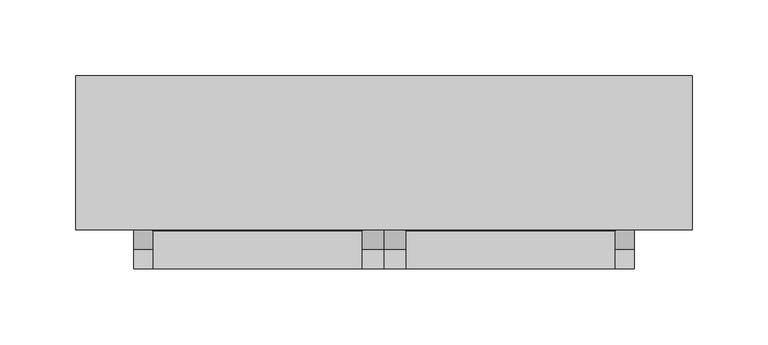
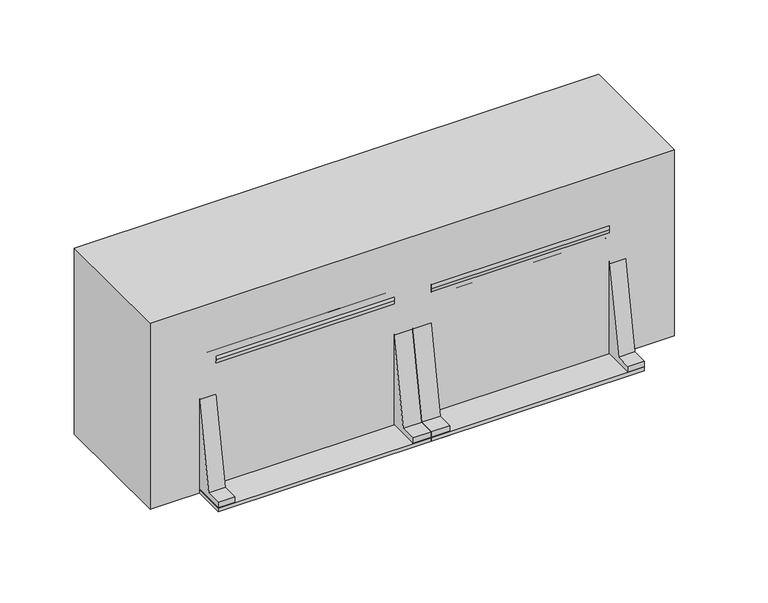
"""IFC4 building model written with IfcOpenShell, lengths in millimetres: proxy geometry, A5202 - Dispenser,Toilet Paper W Utility Shelf, SS, 2-Roll : A5202 - Dispenser,Toilet Paper W Utility Shelf, SS, 2-Roll."""

import ifcopenshell
import ifcopenshell.guid

model = None  # the IFC model being written
_history = None  # IfcOwnerHistory: only IFC2X3 demands one
_inside = {}  # id of a spatial element -> (the spatial element, [elements in it])
_under = {}  # id of a project, library or spatial element -> (it, [spatial elements below it])
_declared = {}  # id of a project -> (the project, [libraries it declares])
_typed = {}  # id of a type object -> (the type object, [elements of that type])
_made_of = {}  # id of a material, layer set ... -> (it, [elements and type objects made of it])


def new_model(schema):
    """Start an empty IFC model of exactly this schema.

    Asked for "IFC4X3", IfcOpenShell would pick the latest addendum, in which some entities
    have other attributes; the version numbers below select the first issue.
    IFC2X3 requires an IfcOwnerHistory on every rooted entity: one is made here for all.
    """
    global model, _history
    if schema == "IFC4X3":
        model = ifcopenshell.file(schema_version=(4, 3, 0, 0))
    else:
        model = ifcopenshell.file(schema=schema)
    _inside.clear()
    _under.clear()
    _declared.clear()
    _typed.clear()
    _made_of.clear()
    _history = None
    if model.schema == "IFC2X3":
        org = make("IfcOrganization", Name="unknown")
        user = make(
            "IfcPersonAndOrganization",
            ThePerson=make("IfcPerson", FamilyName="unknown"),
            TheOrganization=org,
        )
        app = make(
            "IfcApplication",
            ApplicationDeveloper=org,
            Version="unknown",
            ApplicationFullName="unknown",
            ApplicationIdentifier="unknown",
        )
        _history = make(
            "IfcOwnerHistory",
            OwningUser=user,
            OwningApplication=app,
            ChangeAction="ADDED",
            CreationDate=0,
        )
    return model


def make(cls, **values):
    """One entity of the class cls with the attributes given. An attribute that is None is left unset."""
    return model.create_entity(
        cls, **{name: value for name, value in values.items() if value is not None}
    )


def rooted(cls, **values):
    """An entity with a GlobalId (a new one), such as an element, a storey or a relation."""
    return make(cls, GlobalId=ifcopenshell.guid.new(), OwnerHistory=_history, **values)


def si_unit(unit_type, name, prefix=None):
    """IfcSIUnit, for example si_unit("LENGTHUNIT", "METRE", prefix="MILLI")."""
    return make("IfcSIUnit", UnitType=unit_type, Prefix=prefix, Name=name)


def assignment(units):
    """IfcUnitAssignment: the units of a project."""
    return None if units is None else make("IfcUnitAssignment", Units=units)


def point(xyz):
    """IfcCartesianPoint."""
    return None if xyz is None else make("IfcCartesianPoint", Coordinates=xyz)


def direction(xyz):
    """IfcDirection."""
    return None if xyz is None else make("IfcDirection", DirectionRatios=xyz)


def frame(location, z_axis=None, x_axis=None):
    """IfcAxis2Placement3D, a coordinate frame: its origin and axes. An axis left out is left unset."""
    return make(
        "IfcAxis2Placement3D",
        Location=point(location),
        Axis=direction(z_axis),
        RefDirection=direction(x_axis),
    )


def frame_2d(location, x_axis=None):
    """IfcAxis2Placement2D, a coordinate frame in the plane: its origin and x axis."""
    return make(
        "IfcAxis2Placement2D", Location=point(location), RefDirection=direction(x_axis)
    )


def origin():
    """The frame at (0, 0, 0) with its axes left unset."""
    return frame((0.0, 0.0, 0.0))


def origin_with_axes():
    """The frame at (0, 0, 0) with the z axis (0, 0, 1) and the x axis (1, 0, 0) written out."""
    return frame((0.0, 0.0, 0.0), z_axis=(0.0, 0.0, 1.0), x_axis=(1.0, 0.0, 0.0))


def place(relative_to, where):
    """IfcLocalPlacement: puts the frame where relative to a parent placement (None: the world)."""
    return make(
        "IfcLocalPlacement", PlacementRelTo=relative_to, RelativePlacement=where
    )


def context(
    kind, dimensions, precision=None, world=None, true_north=None, identifier=None
):
    """IfcGeometricRepresentationContext, for example the 3D "Model" context."""
    return make(
        "IfcGeometricRepresentationContext",
        ContextIdentifier=identifier,
        ContextType=kind,
        CoordinateSpaceDimension=dimensions,
        Precision=precision,
        WorldCoordinateSystem=world,
        TrueNorth=true_north,
    )


def project(units=None, contexts=None):
    """IfcProject with its units and contexts."""
    return rooted(
        "IfcProject",
        Name="project",
        RepresentationContexts=contexts,
        UnitsInContext=assignment(units),
    )


def spatial(cls, under=None, at=None, **own):
    """A site, building, storey or space (cls), placed at a placement, below another one or the project."""
    s = rooted(cls, ObjectPlacement=at, **own)
    if under is not None:
        _under.setdefault(under.id(), (under, []))[1].append(s)
    return s


def polyline(points):
    """IfcPolyline through the points."""
    return make("IfcPolyline", Points=[point(p) for p in points])


def circle_curve(where, radius):
    """IfcCircle in the frame where."""
    return make("IfcCircle", Position=where, Radius=radius)


def trimmed(basis, trim1, trim2, sense, master):
    """IfcTrimmedCurve: the piece of a basis curve between two trims."""
    return make(
        "IfcTrimmedCurve",
        BasisCurve=basis,
        Trim1=trim1,
        Trim2=trim2,
        SenseAgreement=sense,
        MasterRepresentation=master,
    )


def segment(curve, same_sense, transition):
    """IfcCompositeCurveSegment."""
    return make(
        "IfcCompositeCurveSegment",
        Transition=transition,
        SameSense=same_sense,
        ParentCurve=curve,
    )


def composite_curve(segments, self_intersect=None):
    """IfcCompositeCurve: segments joined end to end."""
    return make("IfcCompositeCurve", Segments=segments, SelfIntersect=self_intersect)


def outline(outer, holes=None, kind="AREA"):
    """IfcArbitraryClosedProfileDef: a profile drawn as a closed curve; with holes, ...WithVoids."""
    if holes is None:
        return make("IfcArbitraryClosedProfileDef", ProfileType=kind, OuterCurve=outer)
    return make(
        "IfcArbitraryProfileDefWithVoids",
        ProfileType=kind,
        OuterCurve=outer,
        InnerCurves=holes,
    )


def extrude(swept, where, along, depth):
    """IfcExtrudedAreaSolid: the profile swept, set in the frame where, extruded along a direction by depth."""
    return make(
        "IfcExtrudedAreaSolid",
        SweptArea=swept,
        Position=where,
        ExtrudedDirection=direction(along),
        Depth=depth,
    )


def faces_of(points, faces, orient=None, outer=None):
    """IfcFace entities. A face is a list of loops; a loop is a list of indices into points, from 0.

    orient and outer hold one flag for each loop. By default every Orientation is true, the
    first loop of a face is its IfcFaceOuterBound and the others are IfcFaceBound.
    """
    made = []
    for i, loops in enumerate(faces):
        bounds = []
        for j, loop in enumerate(loops):
            is_outer = j == 0 if outer is None else outer[i][j]
            bounds.append(
                make(
                    "IfcFaceOuterBound" if is_outer else "IfcFaceBound",
                    Bound=make("IfcPolyLoop", Polygon=[points[k] for k in loop]),
                    Orientation=True if orient is None else orient[i][j],
                )
            )
        made.append(make("IfcFace", Bounds=bounds))
    return made


def faceted_brep(points, faces, orient=None, outer=None, voids=None):
    """IfcFacetedBrep: a solid bounded by flat faces; with voids (closed shells), ...WithVoids."""
    shared = [point(p) for p in points]
    hull = make("IfcClosedShell", CfsFaces=faces_of(shared, faces, orient, outer))
    if voids is None:
        return make("IfcFacetedBrep", Outer=hull)
    return make(
        "IfcFacetedBrepWithVoids",
        Outer=hull,
        Voids=[
            make(cls, CfsFaces=faces_of(shared, fs, o, b)) for cls, fs, o, b in voids
        ],
    )


def shape(context_of_items, identifier, shape_type, items):
    """IfcShapeRepresentation: the items that make up one representation, for example the "Body"."""
    return make(
        "IfcShapeRepresentation",
        ContextOfItems=context_of_items,
        RepresentationIdentifier=identifier,
        RepresentationType=shape_type,
        Items=items,
    )


def source(mapping_origin, context_of_items, identifier, shape_type, items):
    """IfcRepresentationMap: a shape defined once, which mapped items show again and again."""
    return make(
        "IfcRepresentationMap",
        MappingOrigin=mapping_origin,
        MappedRepresentation=shape(context_of_items, identifier, shape_type, items),
    )


def transform(
    local_origin,
    x_axis=None,
    y_axis=None,
    z_axis=None,
    scale=None,
    scale2=None,
    scale3=None,
    uniform=True,
):
    """IfcCartesianTransformationOperator3D, or its non-uniform kind. x_axis, y_axis, z_axis: its Axis1, 2, 3."""
    if uniform:
        return make(
            "IfcCartesianTransformationOperator3D",
            Axis1=direction(x_axis),
            Axis2=direction(y_axis),
            LocalOrigin=point(local_origin),
            Scale=scale,
            Axis3=direction(z_axis),
        )
    return make(
        "IfcCartesianTransformationOperator3DnonUniform",
        Axis1=direction(x_axis),
        Axis2=direction(y_axis),
        LocalOrigin=point(local_origin),
        Scale=scale,
        Axis3=direction(z_axis),
        Scale2=scale2,
        Scale3=scale3,
    )


def mapped(mapping_source, mapping_target):
    """IfcMappedItem: shows the shape of a source again, moved by a transform."""
    return make(
        "IfcMappedItem", MappingSource=mapping_source, MappingTarget=mapping_target
    )


def made_of(thing, what):
    """Note that an element or type object is made of a material, layer set ...; save() writes the relation."""
    if what is not None:
        _made_of.setdefault(what.id(), (what, []))[1].append(thing)
    return thing


def element(
    cls,
    number,
    at=None,
    inside=None,
    cuts=None,
    type_object=None,
    material=None,
    context=None,
    identifier="Body",
    shape_type=None,
    held_by="IfcProductDefinitionShape",
    body=None,
    shapes=None,
    **own,
):
    """One element of the class cls, such as IfcWall. Its Tag is "e" and its number.

    at: its placement. inside: the storey or other place that contains it. cuts: it is an
    opening in that element (IfcRelVoidsElement). A single representation is given by context,
    identifier, shape_type and body (its items); several are given by shapes. held_by: the class
    of the entity that holds the representations. save() writes the other relations.
    """
    e = rooted(cls, Tag="e%d" % number, ObjectPlacement=at, **own)
    if body is not None:
        shapes = [shape(context, identifier, shape_type, body)]
    if shapes is not None:
        e.Representation = make(held_by, Representations=shapes)
    if inside is not None:
        _inside.setdefault(inside.id(), (inside, []))[1].append(e)
    if cuts is not None:
        rooted(
            "IfcRelVoidsElement", RelatingBuildingElement=cuts, RelatedOpeningElement=e
        )
    if type_object is not None:
        _typed.setdefault(type_object.id(), (type_object, []))[1].append(e)
    return made_of(e, material)


def aggregate(whole, parts):
    """IfcRelAggregates: a whole, such as a stair, and the parts it consists of."""
    return rooted("IfcRelAggregates", RelatingObject=whole, RelatedObjects=parts)


def save(model, path):
    """Write the relations noted so far, then the file.

    IfcRelAggregates (storeys below a building ...), IfcRelContainedInSpatialStructure (elements
    in a storey), IfcRelDefinesByType, IfcRelAssociatesMaterial and IfcRelDeclares: one each for
    every whole, place, type object, material and project.
    """
    for whole, parts in _under.values():
        aggregate(whole, parts)
    for where, things in _inside.values():
        rooted(
            "IfcRelContainedInSpatialStructure",
            RelatedElements=things,
            RelatingStructure=where,
        )
    for kind, things in _typed.values():
        rooted("IfcRelDefinesByType", RelatedObjects=things, RelatingType=kind)
    for what, things in _made_of.values():
        rooted("IfcRelAssociatesMaterial", RelatedObjects=things, RelatingMaterial=what)
    for by, libraries in _declared.values():
        rooted("IfcRelDeclares", RelatingContext=by, RelatedDefinitions=libraries)
    model.write(path)


def specialty_equipment_d6a35412(model_context):
    return source(origin(), model_context, "Body", "SolidModel", [
        extrude(outline(polyline([(203.2, 0.0), (203.2, -101.6), (-203.2, -101.6), (-203.2, 0.0), (203.2, 0.0)])), origin_with_axes(), (0.0, 0.0, 1.0), 152.4),
        faceted_brep([(152.4, -3.175, 3.175), (-152.4, -3.175, 3.175), (-152.4, -12.7, 3.175), (152.4, -12.7, 3.175), (165.1, -12.7, 149.225), (165.1, 0.0, 149.225), (-165.1, 0.0, 149.225), (-165.1, -12.7, 149.225), (165.1, -12.7, 0.0), (-165.1, -12.7, 0.0), (-165.1, 0.0, 0.0), (165.1, 0.0, 0.0), (-152.4, -12.7, 145.6205323), (152.4, -12.7, 145.6205323), (152.4, -3.175, 145.6205323), (-152.4, -3.175, 145.6205323)], [[[0, 1, 2, 3]], [[4, 5, 6, 7]], [[8, 9, 10, 11]], [[5, 4, 8, 11]], [[6, 5, 11, 10]], [[7, 6, 10, 9]], [[4, 7, 9, 8], [12, 13, 3, 2]], [[14, 15, 1, 0]], [[15, 14, 13, 12]], [[1, 15, 12, 2]], [[14, 0, 3, 13]]]),
        extrude(outline(polyline([(0.0, -12.7), (165.1, -12.7), (165.1, -127.2036203), (0.0, -127.2036203), (0.0, -12.7)])), origin_with_axes(), (0.0, 0.0, 1.0), 3.175),
        extrude(outline(polyline([(-124.0286203, 0.0), (0.0, 0.0), (0.0, -7.9375), (-12.7, -7.9375), (-33.2613189, -120.65), (-114.5036203, -120.65), (-114.5036203, -3.175), (-124.0286203, -3.175), (-124.0286203, 0.0)])), frame((0.0, -127.2036203, 0.0), z_axis=(1.0, 1.020266240683039e-12, 0.0), x_axis=(1.020266240683039e-12, -1.0, 0.0)), (0.0, 0.0, 1.0), 14.2875),
        extrude(outline(polyline([(-114.5036203, 0.0), (0.0, 0.0), (0.0, -7.9375), (-12.7, -7.9375), (-33.2613189, -120.65), (-114.5036203, -120.65), (-114.5036203, 0.0)])), frame((152.4, -127.2036203, 0.0), z_axis=(1.0, 1.020266240683039e-12, 0.0), x_axis=(1.020266240683039e-12, -1.0, 0.0)), (0.0, 0.0, 1.0), 12.7),
        extrude(outline(polyline([(0.0, -12.7), (0.0, -127.2036203), (-165.1, -127.2036203), (-165.1, -12.7), (0.0, -12.7)])), origin_with_axes(), (0.0, 0.0, 1.0), 3.175),
        extrude(outline(polyline([(0.0, 0.0), (0.0, -124.0286203), (-7.9375, -124.0286203), (-7.9375, -111.3286203), (-120.65, -90.7673014), (-120.65, -9.525), (-3.175, -9.525), (-3.175, 0.0), (0.0, 0.0)])), frame((-14.2875, -3.175, 0.0), z_axis=(1.0, 1.0170616637688368e-12, 0.0), x_axis=(0.0, 0.0, -1.0)), (0.0, 0.0, 1.0), 14.2875),
        extrude(outline(polyline([(0.0, 0.0), (0.0, -114.5036203), (-7.9375, -114.5036203), (-7.9375, -101.8036203), (-120.65, -81.2423014), (-120.65, 0.0), (0.0, 0.0)])), frame((-165.1, -12.7, 0.0), z_axis=(1.0, 1.0170616637688368e-12, 0.0), x_axis=(0.0, 0.0, -1.0)), (0.0, 0.0, 1.0), 12.7),
        extrude(outline(composite_curve([segment(trimmed(circle_curve(frame_2d((0.0, -13.382926)), 13.382926), [point((0.0, -26.765852))], [point((0.0, 0.0))], False, "CARTESIAN"), True, "CONTINUOUS"), segment(trimmed(circle_curve(frame_2d((0.0, -13.382926)), 13.382926), [point((0.0, 0.0))], [point((0.0, -26.765852))], False, "CARTESIAN"), True, "CONTINUOUS")], self_intersect=False)), frame((14.2875, -75.517074, 105.1171268), z_axis=(1.0, 1.020266240683039e-12, 0.0), x_axis=(0.0, 0.0, -1.0)), (0.0, 0.0, 1.0), 138.1125),
        extrude(outline(composite_curve([segment(trimmed(circle_curve(frame_2d((0.0, -1.8851296)), 1.8851296), [point((0.0, -3.7702592))], [point((0.0, 0.0))], False, "CARTESIAN"), True, "CONTINUOUS"), segment(trimmed(circle_curve(frame_2d((0.0, -1.8851296)), 1.8851296), [point((0.0, 0.0))], [point((0.0, -3.7702592))], False, "CARTESIAN"), True, "CONTINUOUS")], self_intersect=False)), frame((14.2875, -88.9, 107.0022564), z_axis=(1.0, 1.018725182543629e-12, 0.0), x_axis=(-1.018725182543629e-12, 1.0, 0.0)), (0.0, 0.0, 1.0), 138.1125),
        extrude(outline(composite_curve([segment(trimmed(circle_curve(frame_2d((0.0, -13.382926)), 13.382926), [point((0.0, -26.765852))], [point((0.0, 0.0))], False, "CARTESIAN"), True, "CONTINUOUS"), segment(trimmed(circle_curve(frame_2d((0.0, -13.382926)), 13.382926), [point((0.0, 0.0))], [point((0.0, -26.765852))], False, "CARTESIAN"), True, "CONTINUOUS")], self_intersect=False)), frame((-152.4, -75.517074, 105.1171268), z_axis=(1.0, 1.0170616637688368e-12, 0.0), x_axis=(0.0, 0.0, -1.0)), (0.0, 0.0, 1.0), 138.1125),
        extrude(outline(composite_curve([segment(trimmed(circle_curve(frame_2d((0.0, -1.8851296)), 1.8851296), [point((0.0, -3.7702592))], [point((0.0, 0.0))], False, "CARTESIAN"), True, "CONTINUOUS"), segment(trimmed(circle_curve(frame_2d((0.0, -1.8851296)), 1.8851296), [point((0.0, 0.0))], [point((0.0, -3.7702592))], False, "CARTESIAN"), True, "CONTINUOUS")], self_intersect=False)), frame((-152.4, -88.9, 107.0022564), z_axis=(1.0, 1.0186027219082467e-12, 0.0), x_axis=(-1.0186027219082467e-12, 1.0, 0.0)), (0.0, 0.0, 1.0), 138.1125),
    ])


if __name__ == "__main__":
    model = new_model("IFC4")
    model_context = context("Model", 3, world=origin())
    ifc_project = project(units=[si_unit("LENGTHUNIT", "METRE", prefix="MILLI")], contexts=[model_context])
    site = spatial("IfcSite", under=ifc_project)
    building = spatial("IfcBuilding", under=site)
    placement = place(None, origin())
    specialty_equipment_shape = specialty_equipment_d6a35412(model_context)
    element("IfcBuildingElementProxy", 1, Name="A5202 - Dispenser,Toilet Paper W Utility Shelf, SS, 2-Roll : A5202 - Dispenser,Toilet Paper W Utility Shelf, SS, 2-Roll", ObjectType="A5202 - Dispenser,Toilet Paper W Utility Shelf, SS, 2-Roll : A5202 - Dispenser,Toilet Paper W Utility Shelf, SS, 2-Roll", at=placement, inside=building, context=model_context, shape_type="MappedRepresentation", body=[
        mapped(specialty_equipment_shape, transform((0.0, 0.0, 0.0), x_axis=(1.0, 0.0, 0.0), y_axis=(0.0, 1.0, 0.0), z_axis=(0.0, 0.0, 1.0))),
    ])
    save(model, "model.ifc")

# Revit data of these elements
# Type "A5202 - Dispenser,Toilet Paper W Utility Shelf, SS, 2-Roll : A5202 - Dispenser,Toilet Paper W Utility Shelf, SS, 2-Roll"
#   Watts2 = "0"
#   Watts1 = "0"
#   Unit_Issue = "EA"
#   UTIL_6_Misc = "-"
#   UTIL_5_NonMedGas = "-"
#   UTIL_4_MiscGas = "-"
#   UTIL_3_MedGas = "-"
#   UTIL_2_Elec = "-"
#   UTIL_1_WaterDrain = "-"
#   Nomenclature = "Dispenser,Toilet Paper w/Utility Shelf, SS, 2-Roll"
#   NSN = "4510"
#   Location [instance default] = ""
#   JSN = "A5202"
#   Fund_Source_VA = "-"
#   Fund_Source_Navy = "-"
#   Fund_Source_Army = "-"
#   Fund_Source_AF = "-"
#   ELEC_Volts2 = "0"
#   ELEC_Volts1 = "0"
#   ELEC_Phase2 = "0"
#   ELEC_Phase1 = "0"
#   ELEC_HertzSwitch = "0"
#   ELEC_HertzDependent = "0"
#   ELEC_Hertz = "0"
#   ELEC_Amps2 = "0"
#   ELEC_Amps1 = "0"
#   DetailDescription = "A concealed surface mounted, double roll, satin finish stainless steel, combination toilet tissue dispenser and utility shelf (minimum 5\" depth). Unit accommodates two standard-core toilet tissue rolls through 6\" in diameter. Spindles are chrome plated plastic with a heavyduty internal spring and turn freely for non-controlled delivery. For general purpose use in restrooms."
#   CAT_VA = "A"
#   CAT_Navy = "A"
#   CAT_IHS = "-"
#   CAT_Army = "A"
#   CAT_AF = "A"
#   BTUperhour = "0"
#   Weight_IP = 4
#   Default Elevation = 2' - 0"
#   DIM_Width_IP = 1' - 4"
#   DIM_Height_IP = 0' - 4"
#   DIM_Depth_IP = 0' - 6"
#   Assembly Code = ""
# Element 1 (IfcBuildingElementProxy, "A5202 - Dispenser,Toilet Paper W Utility Shelf, SS, 2-Roll : A5202 - Dispenser,Toilet Paper W Utility Shelf, SS, 2-Roll")
#   Location = "TLTU1"
#   Materials on its faces: "American Specialties - Toilet Tissue Dispenser - Satin Matte", "American Specialties - Toilet Tissue Dispenser - Gray Plastic", "EquipSpace"
# Materials
#   "American Specialties - Toilet Tissue Dispenser - Satin Matte": class "Metal", colour RGB 168 168 168, transparency 0, Model = "0264-1", Manufacturer = "American Specialties", URL = "http://www.americanspecialties.com/new_website/toilet-paper.htm", Description = "Heavy duty cast aluminum, satin finish", Cost = 0
#   "American Specialties - Toilet Tissue Dispenser - Gray Plastic": class "Plastic", colour RGB 85 85 85, transparency 0, Model = "0264-1", Manufacturer = "American Specialties", URL = "http://www.americanspecialties.com/new_website/toilet-paper.htm", Description = "Plastic Spindles", Cost = 0
#   "EquipSpace": class "Unassigned", colour RGB 221 217 195, transparency 0.5
